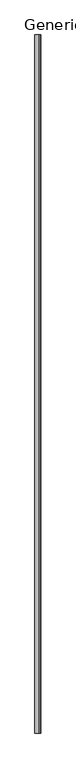
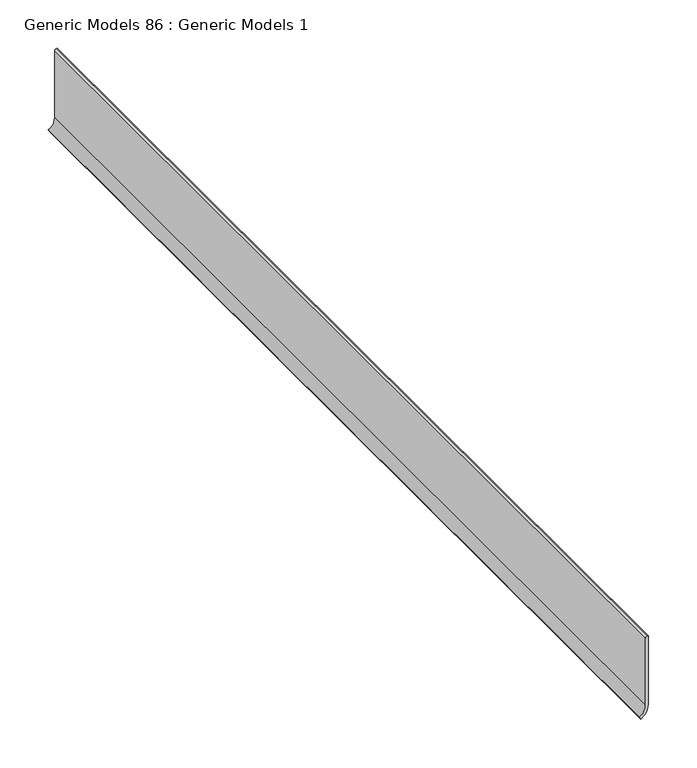
"""IFC4 building model written with IfcOpenShell, lengths in millimetres: proxy geometry, Generic Models 86 : Generic Models 1."""

from ifc_helpers import new_model, si_unit, point, frame, frame_2d, origin, place, context, project, spatial, polyline, circle_curve, trimmed, segment, composite_curve, outline, extrude, source, transform, mapped, element, save


def generic_models_86_generic_models_1_e8e5dea3(model_context):
    return source(origin(), model_context, "Body", "SweptSolid", [
        extrude(outline(composite_curve([segment(polyline([(101.6, 48367.3939813), (101.6, 48366.3057831)]), True, "CONTINUOUS"), segment(trimmed(circle_curve(frame_2d((99.5131982, 48366.3057831)), 2.0868018), [point((101.6, 48366.3057831))], [point((99.5131982, 48364.2189813))], False, "CARTESIAN"), True, "CONTINUOUS"), segment(polyline([(99.5131982, 48364.2189813), (15.4496307, 48364.2189813)]), True, "CONTINUOUS"), segment(trimmed(circle_curve(frame_2d((15.4496307, 48349.5542845)), 14.6646968), [point((15.4496307, 48364.2189813))], [point((2.7496307, 48356.8866329))], True, "CARTESIAN"), True, "CONTINUOUS"), segment(polyline([(2.7496307, 48356.8866329), (0.0, 48358.4741329)]), True, "CONTINUOUS"), segment(trimmed(circle_curve(frame_2d((15.4496307, 48349.5542845)), 17.8396968), [point((0.0, 48358.4741329))], [point((15.4496307, 48367.3939813))], False, "CARTESIAN"), True, "CONTINUOUS"), segment(polyline([(15.4496307, 48367.3939813), (101.6, 48367.3939813)]), True, "CONTINUOUS")], self_intersect=False)), frame((0.0, 0.0, 0.0), z_axis=(0.0, 1.0, 0.0), x_axis=(0.0, 0.0, 1.0)), (0.0, 0.0, 1.0), 1219.2),
    ])


if __name__ == "__main__":
    model = new_model("IFC4")
    model_context = context("Model", 3, world=origin())
    ifc_project = project(units=[si_unit("LENGTHUNIT", "METRE", prefix="MILLI")], contexts=[model_context])
    site = spatial("IfcSite", under=ifc_project)
    building = spatial("IfcBuilding", under=site)
    placement = place(None, origin())
    generic_models_86_generic_models_1_shape = generic_models_86_generic_models_1_e8e5dea3(model_context)
    element("IfcBuildingElementProxy", 1, Name="Generic Models 86 : Generic Models 1", ObjectType="Generic Models 86 : Generic Models 1", at=placement, inside=building, context=model_context, shape_type="MappedRepresentation", body=[
        mapped(generic_models_86_generic_models_1_shape, transform((0.0, 0.0, 0.0), x_axis=(1.0, 0.0, 0.0), y_axis=(0.0, 1.0, 0.0), z_axis=(0.0, 0.0, 1.0))),
    ])
    save(model, "model.ifc")

# Revit data of these elements
# Element 1 (IfcBuildingElementProxy, "Generic Models 86 : Generic Models 1")
#   Materials on its faces: "BASE AS SCHEDULED"
# Materials
#   "BASE AS SCHEDULED": class "Generic", colour RGB 120 120 120, transparency 0, Cost = 0
